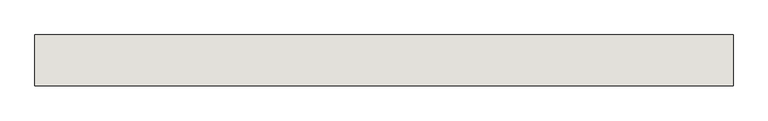
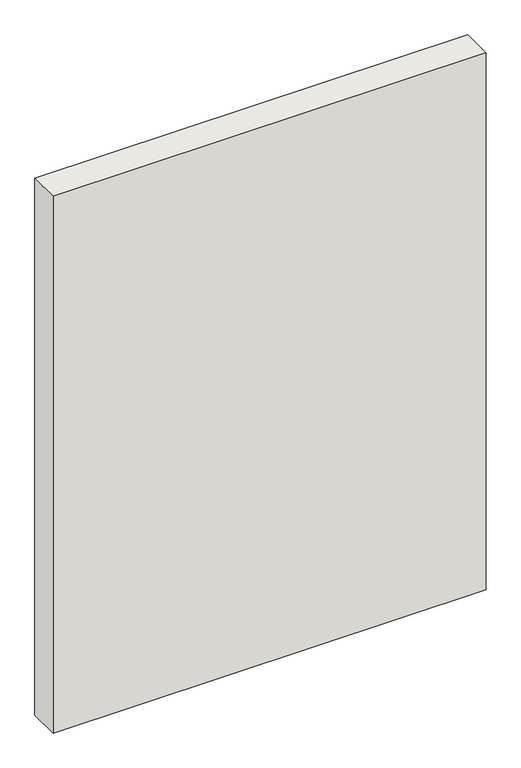
"""IFC4 building model written with IfcOpenShell, lengths in millimetres: wall geometry, Holzwand."""

from ifc_helpers import new_model, si_unit, origin, origin_with_axes, place, context, project, spatial, polyline, outline, extrude, source, transform, mapped, element, save


def wall_e369781e(model_context):
    return source(origin(), model_context, "Body", "SweptSolid", [
        extrude(outline(polyline([(2199.6864914, 160.0), (2199.6864914, 0.0), (0.0, 0.0), (0.0, 160.0), (2199.6864914, 160.0)])), origin_with_axes(), (0.0, 0.0, 1.0), 2880.0),
    ])


if __name__ == "__main__":
    model = new_model("IFC4")
    model_context = context("Model", 3, world=origin())
    ifc_project = project(units=[si_unit("LENGTHUNIT", "METRE", prefix="MILLI")], contexts=[model_context])
    site = spatial("IfcSite", under=ifc_project)
    building = spatial("IfcBuilding", under=site)
    placement = place(None, origin())
    wall_shape = wall_e369781e(model_context)
    element("IfcWall", 1, ObjectType="Holzwand", at=placement, inside=building, context=model_context, shape_type="MappedRepresentation", body=[
        mapped(wall_shape, transform((0.0, 0.0, 0.0), x_axis=(1.0, 0.0, 0.0), y_axis=(0.0, 1.0, 0.0), z_axis=(0.0, 0.0, 1.0))),
    ])
    save(model, "model.ifc")

# Revit data of these elements
# Element 1 (IfcWall, "Holzwand")
#   Materials on its faces: "holzschalung"
# Materials
#   "holzschalung": class "Unassigned", colour RGB 128 128 128, transparency 0
